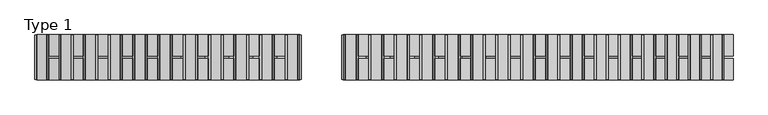
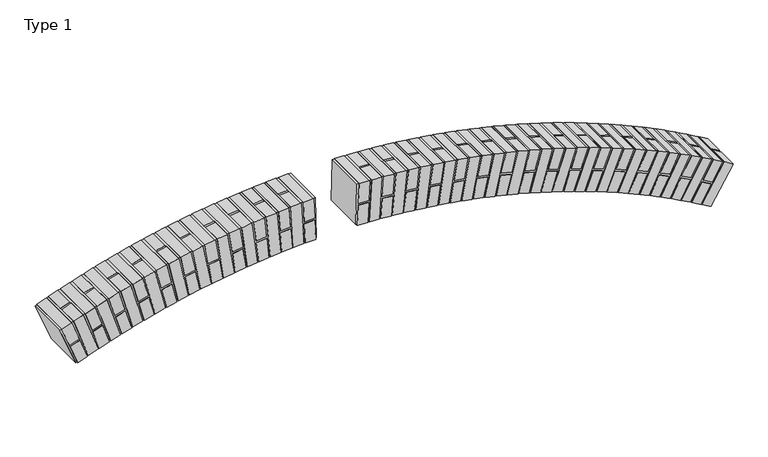
"""IFC4 building model written with IfcOpenShell, lengths in millimetres: proxy geometry, 00_GM_toog : Type 1."""

from ifc_helpers import new_model, si_unit, frame, origin, place, context, project, spatial, polyline, outline, extrude, source, transform, mapped, element, save


def type_1_8e1217ef(model_context):
    return source(origin(), model_context, "Body", "SweptSolid", [
        extrude(outline(polyline([(-33.5304655, 169.1537184), (-33.3801263, 159.6073904), (-133.2870305, 155.2934022), (-131.1300364, 105.3399501), (-31.2231322, 109.6539383), (-30.8114489, 100.1198354), (-235.8183922, 94.5699935), (-236.1881102, 100.8035341), (-141.1349511, 104.9079371), (-143.2919452, 154.8613892), (-237.8024787, 150.7804168), (-238.1723291, 157.0161892), (-33.5304655, 169.1537184)])), frame((0.0, 2.5, 0.0), z_axis=(0.0, 1.0, 0.0), x_axis=(0.0, 0.0, 1.0)), (0.0, 0.0, 1.0), 205.0),
        extrude(outline(polyline([(0.0, 50.0), (210.0, 50.0), (210.0, 0.0), (0.0, 0.0), (0.0, 50.0)])), frame((105.3399501, 210.0, -131.1300364), z_axis=(0.04313988139115512, 0.0, 0.9990690419753567), x_axis=(0.0, -1.0, 0.0)), (0.0, 0.0, 1.0), 100.0),
        extrude(outline(polyline([(0.0, 50.0), (210.0, 50.0), (210.0, 0.0), (0.0, 0.0), (0.0, 50.0)])), frame((100.593949, 210.0, -241.0418553), z_axis=(0.04313988139115512, 0.0, 0.9990690419753567), x_axis=(0.0, -1.0, 0.0)), (0.0, 0.0, 1.0), 100.0),
        extrude(outline(polyline([(210.0, 50.0), (210.0, 0.0), (110.0, 0.0), (110.0, 50.0), (210.0, 50.0)])), frame((206.6325287, 0.0, -246.1224192), z_axis=(0.05920702828123627, 0.0, 0.998245725160947), x_axis=(0.0, 1.0, 0.0)), (0.0, 0.0, 1.0), 210.0),
        extrude(outline(polyline([(100.0, 50.0), (100.0, 0.0), (0.0, 0.0), (0.0, 50.0), (100.0, 50.0)])), frame((206.6325287, 0.0, -246.1224192), z_axis=(0.05920702828123627, 0.0, 0.998245725160947), x_axis=(0.0, 1.0, 0.0)), (0.0, 0.0, 1.0), 210.0),
        extrude(outline(polyline([(-40.8857504, 287.9862039), (-40.4283717, 278.449654), (-140.1447749, 270.9237689), (-136.3818323, 221.0655673), (-36.6654292, 228.5914524), (-35.947235, 219.075529), (-240.6695155, 206.9332303), (-241.2395829, 213.1516499), (-146.3676698, 220.3119073), (-150.1306123, 270.1701089), (-244.4609345, 263.0507269), (-245.0312061, 269.271373), (-40.8857504, 287.9862039)])), frame((0.0, 2.5, 0.0), z_axis=(0.0, 1.0, 0.0), x_axis=(0.0, 0.0, 1.0)), (0.0, 0.0, 1.0), 205.0),
        extrude(outline(polyline([(0.0, 50.0), (210.0, 50.0), (210.0, 0.0), (0.0, 0.0), (0.0, 50.0)])), frame((221.0655673, 210.0, -136.3818323), z_axis=(0.0752588505534319, 0.0, 0.9971640313475895), x_axis=(0.0, -1.0, 0.0)), (0.0, 0.0, 1.0), 100.0),
        extrude(outline(polyline([(0.0, 50.0), (210.0, 50.0), (210.0, 0.0), (0.0, 0.0), (0.0, 50.0)])), frame((212.7860223, 210.0, -246.084073), z_axis=(0.0752588505534319, 0.0, 0.9971640313475895), x_axis=(0.0, -1.0, 0.0)), (0.0, 0.0, 1.0), 100.0),
        extrude(outline(polyline([(210.0, 50.0), (210.0, 0.0), (110.0, 0.0), (110.0, 50.0), (210.0, 50.0)])), frame((318.6062653, 0.0, -254.5734006), z_axis=(0.09129119349759061, 0.0, 0.9958242405112387), x_axis=(0.0, 1.0, 0.0)), (0.0, 0.0, 1.0), 210.0),
        extrude(outline(polyline([(100.0, 50.0), (100.0, 0.0), (0.0, 0.0), (0.0, 50.0), (100.0, 50.0)])), frame((318.6062653, 0.0, -254.5734006), z_axis=(0.09129119349759061, 0.0, 0.9958242405112387), x_axis=(0.0, 1.0, 0.0)), (0.0, 0.0, 1.0), 210.0),
        extrude(outline(polyline([(-52.0602176, 406.5205496), (-51.296273, 397.0036505), (-150.7189429, 386.2736598), (-145.3539475, 336.5623248), (-45.9312776, 347.2923156), (-44.907316, 337.8044231), (-249.1329934, 319.0822379), (-249.9028201, 325.279099), (-155.3103699, 335.4877981), (-160.6753652, 385.199133), (-254.7278199, 375.0487119), (-255.4979222, 381.2477916), (-52.0602176, 406.5205496)])), frame((0.0, 2.5, 0.0), z_axis=(0.0, 1.0, 0.0), x_axis=(0.0, 0.0, 1.0)), (0.0, 0.0, 1.0), 205.0),
        extrude(outline(polyline([(0.0, 50.0), (210.0, 50.0), (210.0, 0.0), (0.0, 0.0), (0.0, 50.0)])), frame((336.5623248, 210.0, -145.3539475), z_axis=(0.10729990744537966, 0.0, 0.9942266994313786), x_axis=(0.0, -1.0, 0.0)), (0.0, 0.0, 1.0), 100.0),
        extrude(outline(polyline([(0.0, 50.0), (210.0, 50.0), (210.0, 0.0), (0.0, 0.0), (0.0, 50.0)])), frame((324.7578073, 210.0, -254.7330398), z_axis=(0.10729990744537966, 0.0, 0.9942266994313786), x_axis=(0.0, -1.0, 0.0)), (0.0, 0.0, 1.0), 100.0),
        extrude(outline(polyline([(210.0, 50.0), (210.0, 0.0), (110.0, 0.0), (110.0, 50.0), (210.0, 50.0)])), frame((430.2501625, 0.0, -266.6223426), z_axis=(0.12328084884442252, 0.0, 0.9923718216012578), x_axis=(0.0, 1.0, 0.0)), (0.0, 0.0, 1.0), 210.0),
        extrude(outline(polyline([(100.0, 50.0), (100.0, 0.0), (0.0, 0.0), (0.0, 50.0), (100.0, 50.0)])), frame((430.2501625, 0.0, -266.6223426), z_axis=(0.12328084884442252, 0.0, 0.9923718216012578), x_axis=(0.0, 1.0, 0.0)), (0.0, 0.0, 1.0), 210.0),
        extrude(outline(polyline([(-67.0422986, 524.634042), (-65.9725789, 515.1466462), (-164.9985876, 501.2236581), (-158.0370935, 451.7106537), (-59.0110848, 465.6336418), (-57.6824158, 456.1836027), (-261.2000642, 430.9009134), (-262.1688531, 437.0698005), (-167.9537933, 450.3163726), (-174.9152873, 499.829377), (-268.592506, 486.658425), (-269.5616418, 492.8295207), (-67.0422986, 524.634042)])), frame((0.0, 2.5, 0.0), z_axis=(0.0, 1.0, 0.0), x_axis=(0.0, 0.0, 1.0)), (0.0, 0.0, 1.0), 205.0),
        extrude(outline(polyline([(0.0, 50.0), (210.0, 50.0), (210.0, 0.0), (0.0, 0.0), (0.0, 50.0)])), frame((451.7106537, 210.0, -158.0370935), z_axis=(0.1392298813307013, 0.0, 0.990260087120873), x_axis=(0.0, -1.0, 0.0)), (0.0, 0.0, 1.0), 100.0),
        extrude(outline(polyline([(0.0, 49.9999999), (210.0, 49.9999999), (210.0, 0.0), (0.0, 0.0), (0.0, 49.9999999)])), frame((436.3933845, 210.0, -266.979802), z_axis=(0.1392298813307013, 0.0, 0.990260087120873), x_axis=(0.0, -1.0, 0.0)), (0.0, 0.0, 1.0), 100.0),
        extrude(outline(polyline([(210.0, 50.0), (210.0, 0.0), (110.0, 0.0), (110.0, 50.0), (210.0, 50.0)])), frame((541.44864, 0.0, -282.2567714), z_axis=(0.15514287679925243, 0.0, 0.9878920425726953), x_axis=(0.0, 1.0, 0.0)), (0.0, 0.0, 1.0), 210.0),
        extrude(outline(polyline([(100.0, 50.0), (100.0, 0.0), (0.0, 0.0), (0.0, 50.0), (100.0, 50.0)])), frame((541.44864, 0.0, -282.2567714), z_axis=(0.15514287679925243, 0.0, 0.9878920425726953), x_axis=(0.0, 1.0, 0.0)), (0.0, 0.0, 1.0), 210.0),
        extrude(outline(polyline([(-85.8164831, 642.2044032), (-84.4420957, 632.7563326), (-182.9689258, 615.6547609), (-174.41814, 566.3913459), (-75.8913099, 583.4929175), (-74.2593091, 574.090515), (-276.8582352, 542.2734956), (-278.0249835, 548.4080224), (-184.2848508, 564.6787539), (-192.8356366, 613.9421689), (-286.0406393, 597.7643214), (-287.2078054, 603.9010445), (-85.8164831, 642.2044032)])), frame((0.0, 2.5, 0.0), z_axis=(0.0, 1.0, 0.0), x_axis=(0.0, 0.0, 1.0)), (0.0, 0.0, 1.0), 205.0),
        extrude(outline(polyline([(0.0, 50.0), (210.0, 50.0), (210.0, 0.0), (0.0, 0.0), (0.0, 50.0)])), frame((566.3913459, 210.0, -174.41814), z_axis=(0.17101571647257813, 0.0, 0.9852683008802073), x_axis=(0.0, -1.0, 0.0)), (0.0, 0.0, 1.0), 100.0),
        extrude(outline(polyline([(0.0, 50.0000001), (210.0, 50.0000001), (210.0, 0.0), (0.0, 0.0), (0.0, 50.0000001)])), frame((547.5771822, 210.0, -282.8116809), z_axis=(0.17101571647257813, 0.0, 0.9852683008802073), x_axis=(0.0, -1.0, 0.0)), (0.0, 0.0, 1.0), 100.0),
        extrude(outline(polyline([(210.0, 50.0), (210.0, 0.0), (110.0, 0.0), (110.0, 50.0), (210.0, 50.0)])), frame((652.086579, 0.0, -301.4605014), z_axis=(0.186844291966782, 0.0, 0.982389541149249), x_axis=(0.0, 1.0, 0.0)), (0.0, 0.0, 1.0), 210.0),
        extrude(outline(polyline([(100.0, 50.0), (100.0, 0.0), (0.0, 0.0), (0.0, 50.0), (100.0, 50.0)])), frame((652.086579, 0.0, -301.4605014), z_axis=(0.186844291966782, 0.0, 0.982389541149249), x_axis=(0.0, 1.0, 0.0)), (0.0, 0.0, 1.0), 210.0),
        extrude(outline(polyline([(-108.363335, 759.1099176), (-106.6857028, 749.7109533), (-204.6113536, 729.4485027), (-194.4801283, 680.4856773), (-96.5544775, 700.7481279), (-94.6208344, 691.4030958), (-296.0912962, 653.0846852), (-297.454796, 659.1785008), (-204.2866356, 678.4565473), (-214.4178609, 727.4193728), (-307.0541565, 708.251378), (-308.4181444, 714.3473753), (-108.363335, 759.1099176)])), frame((0.0, 2.5, 0.0), z_axis=(0.0, 1.0, 0.0), x_axis=(0.0, 0.0, 1.0)), (0.0, 0.0, 1.0), 205.0),
        extrude(outline(polyline([(0.0, 50.0), (210.0, 50.0), (210.0, 0.0), (0.0, 0.0), (0.0, 50.0)])), frame((680.4856773, 210.0, -194.4801283), z_axis=(0.20262450635487594, 0.0, 0.9792565084922555), x_axis=(0.0, -1.0, 0.0)), (0.0, 0.0, 1.0), 100.0),
        extrude(outline(polyline([(0.0, 50.0), (210.0, 50.0), (210.0, 0.0), (0.0, 0.0), (0.0, 50.0)])), frame((658.1940967, 210.0, -302.2122865), z_axis=(0.20262450635487594, 0.0, 0.9792565084922555), x_axis=(0.0, -1.0, 0.0)), (0.0, 0.0, 1.0), 100.0),
        extrude(outline(polyline([(210.0, 49.9999999), (210.0, 0.0), (110.0, 0.0), (110.0, 49.9999999), (210.0, 49.9999999)])), frame((762.0494405, 0.0, -324.2136517), z_axis=(0.21835227522726555, 0.0, 0.9758700138353861), x_axis=(0.0, 1.0, 0.0)), (0.0, 0.0, 1.0), 210.0),
        extrude(outline(polyline([(100.0, 49.9999999), (100.0, 0.0), (0.0, 0.0), (0.0, 49.9999999), (100.0, 49.9999999)])), frame((762.0494405, 0.0, -324.2136517), z_axis=(0.21835227522726555, 0.0, 0.9758700138353861), x_axis=(0.0, 1.0, 0.0)), (0.0, 0.0, 1.0), 210.0),
        extrude(outline(polyline([(-134.6595125, 875.229558), (-132.6803722, 865.8894304), (-229.9034656, 842.4870776), (-218.2022892, 793.875531), (-120.9791959, 817.2778837), (-118.7459124, 807.9998966), (-318.8793361, 763.2197642), (-320.4381758, 769.26656), (-227.9384408, 791.5319638), (-239.6396171, 840.1435105), (-331.6113032, 818.0052122), (-333.1707009, 824.0541729), (-134.6595125, 875.229558)])), frame((0.0, 2.5, 0.0), z_axis=(0.0, 1.0, 0.0), x_axis=(0.0, 0.0, 1.0)), (0.0, 0.0, 1.0), 205.0),
        extrude(outline(polyline([(0.0, 49.9999999), (210.0, 49.9999999), (210.0, 0.0), (0.0, 0.0), (0.0, 49.9999999)])), frame((793.875531, 210.0, -218.2022892), z_axis=(0.2340235277488462, 0.0, 0.9722309337086458), x_axis=(0.0, -1.0, 0.0)), (0.0, 0.0, 1.0), 100.0),
        extrude(outline(polyline([(0.0, 50.0), (210.0, 50.0), (210.0, 0.0), (0.0, 0.0), (0.0, 50.0)])), frame((768.129611, 210.0, -325.1615341), z_axis=(0.2340235277488462, 0.0, 0.9722309337086458), x_axis=(0.0, -1.0, 0.0)), (0.0, 0.0, 1.0), 100.0),
        extrude(outline(polyline([(210.0, 50.0), (210.0, 0.0), (110.0, 0.0), (110.0, 50.0), (210.0, 50.0)])), frame((871.2233849, 0.0, -350.492667), z_axis=(0.24963420771274006, 0.0, 0.9683402100189957), x_axis=(0.0, 1.0, 0.0)), (0.0, 0.0, 1.0), 210.0),
        extrude(outline(polyline([(100.0, 50.0), (100.0, 0.0), (0.0, 0.0), (0.0, 50.0), (100.0, 50.0)])), frame((871.2233849, 0.0, -350.492667), z_axis=(0.24963420771274006, 0.0, 0.9683402100189957), x_axis=(0.0, 1.0, 0.0)), (0.0, 0.0, 1.0), 210.0),
        extrude(outline(polyline([(-164.6777923, 990.4431107), (-162.3991929, 981.1714892), (-258.8190779, 954.6534617), (-245.5600642, 906.4435193), (-149.1401792, 932.9615467), (-146.6095673, 923.7602096), (-345.1987634, 872.5647144), (-346.9513291, 878.5582304), (-255.2157805, 903.787941), (-268.4747942, 951.9978835), (-359.6866564, 926.9122005), (-361.4398495, 932.9078623), (-164.6777923, 990.4431107)])), frame((0.0, 2.5, 0.0), z_axis=(0.0, 1.0, 0.0), x_axis=(0.0, 0.0, 1.0)), (0.0, 0.0, 1.0), 205.0),
        extrude(outline(polyline([(0.0, 49.9999999), (210.0, 49.9999999), (210.0, 0.0), (0.0, 0.0), (0.0, 49.9999999)])), frame((906.4435193, 210.0, -245.5600642), z_axis=(0.2651802745900883, 0.0, 0.9641988498065767), x_axis=(0.0, -1.0, 0.0)), (0.0, 0.0, 1.0), 100.0),
        extrude(outline(polyline([(0.0, 50.0), (210.0, 50.0), (210.0, 0.0), (0.0, 0.0), (0.0, 50.0)])), frame((877.2699135, 210.0, -351.6356655), z_axis=(0.2651802745900883, 0.0, 0.9641988498065767), x_axis=(0.0, -1.0, 0.0)), (0.0, 0.0, 1.0), 100.0),
        extrude(outline(polyline([(210.0, 50.0), (210.0, 0.0), (110.0, 0.0), (110.0, 50.0), (210.0, 50.0)])), frame((979.495389, 0.0, -380.2703418), z_axis=(0.2806577045759451, 0.0, 0.9598079249840363), x_axis=(0.0, 1.0, 0.0)), (0.0, 0.0, 1.0), 210.0),
        extrude(outline(polyline([(100.0, 50.0), (100.0, 0.0), (0.0, 0.0), (0.0, 50.0), (100.0, 50.0)])), frame((979.495389, 0.0, -380.2703418), z_axis=(0.2806577045759451, 0.0, 0.9598079249840363), x_axis=(0.0, 1.0, 0.0)), (0.0, 0.0, 1.0), 210.0),
        extrude(outline(polyline([(-198.3870978, 1104.6312999), (-195.8113982, 1095.4377831), (-291.3282554, 1065.8315339), (-276.5251308, 1018.0731053), (-181.0082736, 1047.6793545), (-178.1829531, 1038.5641932), (-375.0223307, 981.0063356), (-376.9668081, 986.940367), (-286.0904158, 1015.1082652), (-300.8935404, 1062.8666938), (-391.2511509, 1034.8595963), (-393.1963244, 1040.7957522), (-198.3870978, 1104.6312999)])), frame((0.0, 2.5, 0.0), z_axis=(0.0, 1.0, 0.0), x_axis=(0.0, 0.0, 1.0)), (0.0, 0.0, 1.0), 205.0),
        extrude(outline(polyline([(0.0, 50.0), (210.0, 50.0), (210.0, 0.0), (0.0, 0.0), (0.0, 50.0)])), frame((1018.0731053, 210.0, -276.5251308), z_axis=(0.2960624916306871, 0.0, 0.9551685720591049), x_axis=(0.0, -1.0, 0.0)), (0.0, 0.0, 1.0), 100.0),
        extrude(outline(polyline([(0.0, 50.0), (210.0, 50.0), (210.0, 0.0), (0.0, 0.0), (0.0, 50.0)])), frame((985.502016, 210.0, -381.607273), z_axis=(0.2960624916306871, 0.0, 0.9551685720591049), x_axis=(0.0, -1.0, 0.0)), (0.0, 0.0, 1.0), 100.0),
        extrude(outline(polyline([(210.0, 50.0), (210.0, 0.0), (110.0, 0.0), (110.0, 50.0), (210.0, 50.0)])), frame((1086.7533633, 0.0, -413.5158485), z_axis=(0.3113906485169718, 0.0, 0.9502819918404114), x_axis=(0.0, 1.0, 0.0)), (0.0, 0.0, 1.0), 210.0),
        extrude(outline(polyline([(100.0, 50.0), (100.0, 0.0), (0.0, 0.0), (0.0, 50.0), (100.0, 50.0)])), frame((1086.7533633, 0.0, -413.5158485), z_axis=(0.3113906485169718, 0.0, 0.9502819918404114), x_axis=(0.0, 1.0, 0.0)), (0.0, 0.0, 1.0), 210.0),
        extrude(outline(polyline([(-235.752531, 1217.6759116), (-232.8823978, 1208.5700171), (-327.3973427, 1175.9061963), (-311.0654323, 1128.6487238), (-216.5504874, 1161.3125446), (-213.4333832, 1152.2929957), (-408.319163, 1088.4323629), (-410.4535391, 1094.3007664), (-320.5303834, 1125.3776912), (-336.8622938, 1172.6351637), (-426.2721093, 1141.7356462), (-428.4072495, 1147.6061507), (-235.752531, 1217.6759116)])), frame((0.0, 2.5, 0.0), z_axis=(0.0, 1.0, 0.0), x_axis=(0.0, 0.0, 1.0)), (0.0, 0.0, 1.0), 205.0),
        extrude(outline(polyline([(0.0, 50.0), (210.0, 50.0), (210.0, 0.0), (0.0, 0.0), (0.0, 50.0)])), frame((1128.6487238, 210.0, -311.0654323), z_axis=(0.32663820783169173, 0.0, 0.945149449126698), x_axis=(0.0, -1.0, 0.0)), (0.0, 0.0, 1.0), 100.0),
        extrude(outline(polyline([(0.0, 50.0), (210.0, 50.0), (210.0, 0.0), (0.0, 0.0), (0.0, 50.0)])), frame((1092.7138704, 210.0, -415.0453283), z_axis=(0.32663820783169173, 0.0, 0.945149449126698), x_axis=(0.0, -1.0, 0.0)), (0.0, 0.0, 1.0), 100.0),
        extrude(outline(polyline([(210.0, 50.0), (210.0, 0.0), (110.0, 0.0), (110.0, 50.0), (210.0, 50.0)])), frame((1192.8862684, 0.0, -450.1947694), z_axis=(0.3418012230329286, 0.0, 0.9397722723794283), x_axis=(0.0, 1.0, 0.0)), (0.0, 0.0, 1.0), 210.0),
        extrude(outline(polyline([(100.0, 50.0), (100.0, 0.0), (0.0, 0.0), (0.0, 50.0), (100.0, 50.0)])), frame((1192.8862684, 0.0, -450.1947694), z_axis=(0.3418012230329286, 0.0, 0.9397722723794283), x_axis=(0.0, 1.0, 0.0)), (0.0, 0.0, 1.0), 210.0),
        extrude(outline(polyline([(-276.7354093, 1329.4599155), (-273.5738137, 1320.4510702), (-366.9889991, 1284.7634932), (-349.1452106, 1238.0559006), (-255.7300253, 1273.7434775), (-252.3243644, 1264.8288786), (-445.0547893, 1194.7315828), (-447.3768545, 1200.528283), (-358.5000292, 1234.4820618), (-376.3438176, 1281.1896545), (-464.7132759, 1247.429706), (-467.0361725, 1253.2284817), (-276.7354093, 1329.4599155)])), frame((0.0, 2.5, 0.0), z_axis=(0.0, 1.0, 0.0), x_axis=(0.0, 0.0, 1.0)), (0.0, 0.0, 1.0), 205.0),
        extrude(outline(polyline([(0.0, 49.9999999), (210.0, 49.9999999), (210.0, 0.0), (0.0, 0.0), (0.0, 49.9999999)])), frame((1238.0559006, 210.0, -349.1452106), z_axis=(0.3568757694613718, 0.0, 0.9341518533789642), x_axis=(0.0, -1.0, 0.0)), (0.0, 0.0, 1.0), 100.0),
        extrude(outline(polyline([(0.0, 50.0), (210.0, 50.0), (210.0, 0.0), (0.0, 0.0), (0.0, 50.0)])), frame((1198.7944849, 210.0, -451.9152145), z_axis=(0.3568757694613718, 0.0, 0.9341518533789642), x_axis=(0.0, -1.0, 0.0)), (0.0, 0.0, 1.0), 100.0),
        extrude(outline(polyline([(210.0, 50.0), (210.0, 0.0), (110.0, 0.0), (110.0, 50.0), (210.0, 50.0)])), frame((1297.7842293, 0.0, -490.2691324), z_axis=(0.3718579453562054, 0.0, 0.9282896468643079), x_axis=(0.0, 1.0, 0.0)), (0.0, 0.0, 1.0), 210.0),
        extrude(outline(polyline([(100.0, 50.0), (100.0, 0.0), (0.0, 0.0), (0.0, 50.0), (100.0, 50.0)])), frame((1297.7842293, 0.0, -490.2691324), z_axis=(0.3718579453562054, 0.0, 0.9282896468643079), x_axis=(0.0, 1.0, 0.0)), (0.0, 0.0, 1.0), 210.0),
        extrude(outline(polyline([(-321.2933048, 1439.8675863), (-317.8435199, 1430.9651168), (-410.0622369, 1392.2907295), (-390.7250433, 1346.181371), (-298.5063263, 1384.8557583), (-294.8156345, 1376.0553381), (-485.1911791, 1299.7939481), (-487.6985293, 1305.512944), (-399.9600447, 1342.308426), (-419.2972383, 1388.4177845), (-506.5348544, 1351.8323552), (-509.0431023, 1357.5533987), (-321.2933048, 1439.8675863)])), frame((0.0, 2.5, 0.0), z_axis=(0.0, 1.0, 0.0), x_axis=(0.0, 0.0, 1.0)), (0.0, 0.0, 1.0), 205.0),
        extrude(outline(polyline([(0.0, 50.0), (210.0, 50.0), (210.0, 0.0), (0.0, 0.0), (0.0, 50.0)])), frame((1346.181371, 210.0, -390.7250433), z_axis=(0.38674387286495593, 0.0, 0.9221871701565875), x_axis=(0.0, -1.0, 0.0)), (0.0, 0.0, 1.0), 100.0),
        extrude(outline(polyline([(0.0, 50.0), (210.0, 50.0), (210.0, 0.0), (0.0, 0.0), (0.0, 50.0)])), frame((1303.6340387, 210.0, -492.1787617), z_axis=(0.38674387286495593, 0.0, 0.9221871701565875), x_axis=(0.0, -1.0, 0.0)), (0.0, 0.0, 1.0), 100.0),
        extrude(outline(polyline([(210.0, 50.0), (210.0, 0.0), (110.0, 0.0), (110.0, 50.0), (210.0, 50.0)])), frame((1401.3386497, 0.0, -533.6974503), z_axis=(0.40152969904724134, 0.0, 0.9158460027663122), x_axis=(0.0, 1.0, 0.0)), (0.0, 0.0, 1.0), 210.0),
        extrude(outline(polyline([(100.0, 50.0), (100.0, 0.0), (0.0, 0.0), (0.0, 50.0), (100.0, 50.0)])), frame((1401.3386497, 0.0, -533.6974503), z_axis=(0.40152969904724134, 0.0, 0.9158460027663122), x_axis=(0.0, 1.0, 0.0)), (0.0, 0.0, 1.0), 210.0),
        extrude(outline(polyline([(-369.3800886, 1548.7846238), (-365.6456858, 1539.9977463), (-456.5724644, 1498.3765867), (-435.7618846, 1452.9131974), (-344.835106, 1494.534357), (-340.8632042, 1485.8572264), (-528.6867806, 1403.5106923), (-531.3768203, 1409.1460633), (-444.8675082, 1448.7451556), (-465.678088, 1494.2085449), (-551.6935484, 1454.8355101), (-554.3845512, 1460.4728988), (-369.3800886, 1548.7846238)])), frame((0.0, 2.5, 0.0), z_axis=(0.0, 1.0, 0.0), x_axis=(0.0, 0.0, 1.0)), (0.0, 0.0, 1.0), 205.0),
        extrude(outline(polyline([(0.0, 50.0), (210.0, 50.0), (210.0, 0.0), (0.0, 0.0), (0.0, 50.0)])), frame((1452.9131974, 210.0, -435.7618846), z_axis=(0.4162115968719885, 0.0, 0.9092677859845631), x_axis=(0.0, -1.0, 0.0)), (0.0, 0.0, 1.0), 100.0),
        extrude(outline(polyline([(0.0, 50.0), (210.0, 50.0), (210.0, 0.0), (0.0, 0.0), (0.0, 50.0)])), frame((1407.1239959, 210.0, -535.7942868), z_axis=(0.4162115968719885, 0.0, 0.9092677859845631), x_axis=(0.0, -1.0, 0.0)), (0.0, 0.0, 1.0), 100.0),
        extrude(outline(polyline([(210.0, 50.0000001), (210.0, 0.0), (110.0, 0.0), (110.0, 50.0000001), (210.0, 50.0000001)])), frame((1503.4423241, 0.0, -580.4347636), z_axis=(0.43078576620803966, 0.0, 0.9024542224581545), x_axis=(0.0, 1.0, 0.0)), (0.0, 0.0, 1.0), 210.0),
        extrude(outline(polyline([(100.0, 50.0000001), (100.0, 0.0), (0.0, 0.0), (0.0, 50.0000001), (100.0, 50.0000001)])), frame((1503.4423241, 0.0, -580.4347636), z_axis=(0.43078576620803966, 0.0, 0.9024542224581545), x_axis=(0.0, 1.0, 0.0)), (0.0, 0.0, 1.0), 210.0),
        extrude(outline(polyline([(-420.9459785, 1656.0982709), (-416.9308239, 1647.4360821), (-506.4715315, 1602.9112386), (-484.2091098, 1558.1408848), (-394.6684022, 1602.6657283), (-390.4194022, 1594.1208702), (-575.4965649, 1505.7744419), (-578.366509, 1511.3203539), (-493.1759289, 1553.6820612), (-515.4383507, 1598.452415), (-600.1426072, 1556.3325361), (-603.0135789, 1561.8804337), (-420.9459785, 1656.0982709)])), frame((0.0, 2.5, 0.0), z_axis=(0.0, 1.0, 0.0), x_axis=(0.0, 0.0, 1.0)), (0.0, 0.0, 1.0), 205.0),
        extrude(outline(polyline([(0.0, 50.0), (210.0, 50.0), (210.0, 0.0), (0.0, 0.0), (0.0, 50.0)])), frame((1558.1408848, 210.0, -484.2091098), z_axis=(0.4452484348076845, 0.0, 0.8954070757489618), x_axis=(0.0, -1.0, 0.0)), (0.0, 0.0, 1.0), 100.0),
        extrude(outline(polyline([(0.0, 49.9999999), (210.0, 49.9999999), (210.0, 0.0), (0.0, 0.0), (0.0, 49.9999999)])), frame((1509.1572178, 210.0, -582.7166365), z_axis=(0.4452484348076845, 0.0, 0.8954070757489618), x_axis=(0.0, -1.0, 0.0)), (0.0, 0.0, 1.0), 100.0),
        extrude(outline(polyline([(210.0, 50.0), (210.0, 0.0), (110.0, 0.0), (110.0, 50.0), (210.0, 50.0)])), frame((1603.9895489, 0.0, -630.4326871), z_axis=(0.4595958592830959, 0.0, 0.8881281698774298), x_axis=(0.0, 1.0, 0.0)), (0.0, 0.0, 1.0), 210.0),
        extrude(outline(polyline([(100.0, 50.0), (100.0, 0.0), (0.0, 0.0), (0.0, 50.0), (100.0, 50.0)])), frame((1603.9895489, 0.0, -630.4326871), z_axis=(0.4595958592830959, 0.0, 0.8881281698774298), x_axis=(0.0, 1.0, 0.0)), (0.0, 0.0, 1.0), 210.0),
        extrude(outline(polyline([(-475.9375905, 1761.6974301), (-471.6458409, 1753.1688977), (-559.7077798, 1705.7864651), (-536.0165635, 1661.7554957), (-447.9546246, 1709.1379283), (-443.4329252, 1700.7341889), (-625.5720717, 1606.4793275), (-628.6189492, 1611.9300392), (-544.8352952, 1657.0105063), (-568.5265115, 1701.0414757), (-651.8318736, 1656.2183574), (-654.879842, 1661.6710206), (-475.9375905, 1761.6974301)])), frame((0.0, 2.5, 0.0), z_axis=(0.0, 1.0, 0.0), x_axis=(0.0, 0.0, 1.0)), (0.0, 0.0, 1.0), 205.0),
        extrude(outline(polyline([(0.0, 50.0), (210.0, 50.0), (210.0, 0.0), (0.0, 0.0), (0.0, 50.0)])), frame((1661.7554957, 210.0, -536.0165635), z_axis=(0.47382432607517866, 0.0, 0.8806193888504856), x_axis=(0.0, -1.0, 0.0)), (0.0, 0.0, 1.0), 100.0),
        extrude(outline(polyline([(0.0, 50.0), (210.0, 50.0), (210.0, 0.0), (0.0, 0.0), (0.0, 50.0)])), frame((1609.6280737, 210.0, -632.8972341), z_axis=(0.47382432607517866, 0.0, 0.8806193888504856), x_axis=(0.0, -1.0, 0.0)), (0.0, 0.0, 1.0), 100.0),
        extrude(outline(polyline([(210.0, 50.0), (210.0, 0.0), (110.0, 0.0), (110.0, 50.0), (210.0, 50.0)])), frame((1702.8762319, 0.0, -683.6394602), z_axis=(0.4879301524148094, 0.0, 0.8728826761738722), x_axis=(0.0, 1.0, 0.0)), (0.0, 0.0, 1.0), 210.0),
        extrude(outline(polyline([(100.0, 50.0), (100.0, 0.0), (0.0, 0.0), (0.0, 50.0), (100.0, 50.0)])), frame((1702.8762319, 0.0, -683.6394602), z_axis=(0.4879301524148094, 0.0, 0.8728826761738722), x_axis=(0.0, 1.0, 0.0)), (0.0, 0.0, 1.0), 210.0),
        extrude(outline(polyline([(-534.2979943, 1865.4727794), (-529.7340926, 1857.0867325), (-616.2260961, 1806.8957638), (-591.1306117, 1763.6497621), (-504.6386083, 1813.8407308), (-499.8488907, 1805.5868102), (-678.86146, 1705.5210939), (-682.0821166, 1710.8709622), (-599.7921264, 1758.6235192), (-624.8876108, 1801.8695209), (-706.7078359, 1754.3895668), (-709.9296455, 1759.7413505), (-534.2979943, 1865.4727794)])), frame((0.0, 2.5, 0.0), z_axis=(0.0, 1.0, 0.0), x_axis=(0.0, 0.0, 1.0)), (0.0, 0.0, 1.0), 205.0),
        extrude(outline(polyline([(0.0, 50.0), (210.0, 50.0), (210.0, 0.0), (0.0, 0.0), (0.0, 50.0)])), frame((1763.6497621, 210.0, -591.1306117), z_axis=(0.5019096872759921, 0.0, 0.864920034349139), x_axis=(0.0, -1.0, 0.0)), (0.0, 0.0, 1.0), 100.0),
        extrude(outline(polyline([(0.0, 50.0), (210.0, 50.0), (210.0, 0.0), (0.0, 0.0), (0.0, 50.0)])), frame((1708.4325505, 210.0, -686.2841298), z_axis=(0.5019096872759921, 0.0, 0.864920034349139), x_axis=(0.0, -1.0, 0.0)), (0.0, 0.0, 1.0), 100.0),
        extrude(outline(polyline([(210.0, 50.0), (210.0, 0.0), (110.0, 0.0), (110.0, 50.0), (210.0, 50.0)])), frame((1800.0, 0.0, -740.0), z_axis=(0.5157593123209204, 0.0, 0.8567335243552988), x_axis=(0.0, 1.0, 0.0)), (0.0, 0.0, 1.0), 210.0),
        extrude(outline(polyline([(100.0, 50.0), (100.0, 0.0), (0.0, 0.0), (0.0, 50.0), (100.0, 50.0)])), frame((1800.0, 0.0, -740.0), z_axis=(0.5157593123209204, 0.0, 0.8567335243552988), x_axis=(0.0, 1.0, 0.0)), (0.0, 0.0, 1.0), 210.0),
        extrude(outline(polyline([(-33.5304655, -169.1537184), (-238.1723291, -157.0161892), (-237.8024787, -150.7804168), (-143.2919452, -154.8613892), (-141.1349511, -104.9079371), (-236.1881102, -100.8035341), (-235.8183922, -94.5699935), (-30.8114489, -100.1198354), (-31.2231322, -109.6539383), (-131.1300364, -105.3399501), (-133.2870305, -155.2934022), (-33.3801263, -159.6073904), (-33.5304655, -169.1537184)])), frame((0.0, 2.5, 0.0), z_axis=(0.0, 1.0, 0.0), x_axis=(0.0, 0.0, 1.0)), (0.0, 0.0, 1.0), 205.0),
        extrude(outline(polyline([(0.0, -50.0), (0.0, 0.0), (210.0, 0.0), (210.0, -50.0), (0.0, -50.0)])), frame((-105.3399501, 210.0, -131.1300364), z_axis=(-0.04313988139115512, 0.0, 0.9990690419753567), x_axis=(0.0, -1.0, 0.0)), (0.0, 0.0, 1.0), 100.0),
        extrude(outline(polyline([(0.0, -50.0), (0.0, 0.0), (210.0, 0.0), (210.0, -50.0), (0.0, -50.0)])), frame((-100.593949, 210.0, -241.0418553), z_axis=(-0.04313988139115512, 0.0, 0.9990690419753567), x_axis=(0.0, -1.0, 0.0)), (0.0, 0.0, 1.0), 100.0),
        extrude(outline(polyline([(210.0, -50.0), (110.0, -50.0), (110.0, 0.0), (210.0, 0.0), (210.0, -50.0)])), frame((-206.6325287, 0.0, -246.1224192), z_axis=(-0.05920702828123627, 0.0, 0.998245725160947), x_axis=(0.0, 1.0, 0.0)), (0.0, 0.0, 1.0), 210.0),
        extrude(outline(polyline([(100.0, -50.0), (0.0, -50.0), (0.0, 0.0), (100.0, 0.0), (100.0, -50.0)])), frame((-206.6325287, 0.0, -246.1224192), z_axis=(-0.05920702828123627, 0.0, 0.998245725160947), x_axis=(0.0, 1.0, 0.0)), (0.0, 0.0, 1.0), 210.0),
        extrude(outline(polyline([(-40.8857504, -287.9862039), (-245.0312061, -269.271373), (-244.4609345, -263.0507269), (-150.1306123, -270.1701089), (-146.3676698, -220.3119073), (-241.2395829, -213.1516499), (-240.6695155, -206.9332303), (-35.947235, -219.075529), (-36.6654292, -228.5914524), (-136.3818323, -221.0655673), (-140.1447749, -270.9237689), (-40.4283717, -278.449654), (-40.8857504, -287.9862039)])), frame((0.0, 2.5, 0.0), z_axis=(0.0, 1.0, 0.0), x_axis=(0.0, 0.0, 1.0)), (0.0, 0.0, 1.0), 205.0),
        extrude(outline(polyline([(0.0, -50.0), (0.0, 0.0), (210.0, 0.0), (210.0, -50.0), (0.0, -50.0)])), frame((-221.0655673, 210.0, -136.3818323), z_axis=(-0.0752588505534319, 0.0, 0.9971640313475895), x_axis=(0.0, -1.0, 0.0)), (0.0, 0.0, 1.0), 100.0),
        extrude(outline(polyline([(0.0, -50.0), (0.0, 0.0), (210.0, 0.0), (210.0, -50.0), (0.0, -50.0)])), frame((-212.7860223, 210.0, -246.084073), z_axis=(-0.0752588505534319, 0.0, 0.9971640313475895), x_axis=(0.0, -1.0, 0.0)), (0.0, 0.0, 1.0), 100.0),
        extrude(outline(polyline([(210.0, -50.0), (110.0, -50.0), (110.0, 0.0), (210.0, 0.0), (210.0, -50.0)])), frame((-318.6062653, 0.0, -254.5734006), z_axis=(-0.09129119349759061, 0.0, 0.9958242405112387), x_axis=(0.0, 1.0, 0.0)), (0.0, 0.0, 1.0), 210.0),
        extrude(outline(polyline([(100.0, -50.0), (0.0, -50.0), (0.0, 0.0), (100.0, 0.0), (100.0, -50.0)])), frame((-318.6062653, 0.0, -254.5734006), z_axis=(-0.09129119349759061, 0.0, 0.9958242405112387), x_axis=(0.0, 1.0, 0.0)), (0.0, 0.0, 1.0), 210.0),
        extrude(outline(polyline([(-52.0602176, -406.5205496), (-255.4979222, -381.2477916), (-254.7278199, -375.0487119), (-160.6753652, -385.199133), (-155.3103699, -335.4877981), (-249.9028201, -325.279099), (-249.1329934, -319.0822379), (-44.907316, -337.8044231), (-45.9312776, -347.2923156), (-145.3539475, -336.5623248), (-150.7189429, -386.2736598), (-51.296273, -397.0036505), (-52.0602176, -406.5205496)])), frame((0.0, 2.5, 0.0), z_axis=(0.0, 1.0, 0.0), x_axis=(0.0, 0.0, 1.0)), (0.0, 0.0, 1.0), 205.0),
        extrude(outline(polyline([(0.0, -50.0), (0.0, 0.0), (210.0, 0.0), (210.0, -50.0), (0.0, -50.0)])), frame((-336.5623248, 210.0, -145.3539475), z_axis=(-0.10729990744537966, 0.0, 0.9942266994313786), x_axis=(0.0, -1.0, 0.0)), (0.0, 0.0, 1.0), 100.0),
        extrude(outline(polyline([(0.0, -50.0), (0.0, 0.0), (210.0, 0.0), (210.0, -50.0), (0.0, -50.0)])), frame((-324.7578073, 210.0, -254.7330398), z_axis=(-0.10729990744537966, 0.0, 0.9942266994313786), x_axis=(0.0, -1.0, 0.0)), (0.0, 0.0, 1.0), 100.0),
        extrude(outline(polyline([(210.0, -50.0), (110.0, -50.0), (110.0, 0.0), (210.0, 0.0), (210.0, -50.0)])), frame((-430.2501625, 0.0, -266.6223426), z_axis=(-0.12328084884442252, 0.0, 0.9923718216012578), x_axis=(0.0, 1.0, 0.0)), (0.0, 0.0, 1.0), 210.0),
        extrude(outline(polyline([(100.0, -50.0), (0.0, -50.0), (0.0, 0.0), (100.0, 0.0), (100.0, -50.0)])), frame((-430.2501625, 0.0, -266.6223426), z_axis=(-0.12328084884442252, 0.0, 0.9923718216012578), x_axis=(0.0, 1.0, 0.0)), (0.0, 0.0, 1.0), 210.0),
        extrude(outline(polyline([(-67.0422986, -524.634042), (-269.5616418, -492.8295207), (-268.592506, -486.658425), (-174.9152873, -499.829377), (-167.9537933, -450.3163726), (-262.1688531, -437.0698005), (-261.2000642, -430.9009134), (-57.6824158, -456.1836027), (-59.0110848, -465.6336418), (-158.0370935, -451.7106537), (-164.9985876, -501.2236581), (-65.9725789, -515.1466462), (-67.0422986, -524.634042)])), frame((0.0, 2.5, 0.0), z_axis=(0.0, 1.0, 0.0), x_axis=(0.0, 0.0, 1.0)), (0.0, 0.0, 1.0), 205.0),
        extrude(outline(polyline([(0.0, -50.0), (0.0, 0.0), (210.0, 0.0), (210.0, -50.0), (0.0, -50.0)])), frame((-451.7106537, 210.0, -158.0370935), z_axis=(-0.1392298813307013, 0.0, 0.990260087120873), x_axis=(0.0, -1.0, 0.0)), (0.0, 0.0, 1.0), 100.0),
        extrude(outline(polyline([(0.0, -49.9999999), (0.0, 0.0), (210.0, 0.0), (210.0, -49.9999999), (0.0, -49.9999999)])), frame((-436.3933845, 210.0, -266.979802), z_axis=(-0.1392298813307013, 0.0, 0.990260087120873), x_axis=(0.0, -1.0, 0.0)), (0.0, 0.0, 1.0), 100.0),
        extrude(outline(polyline([(210.0, -50.0), (110.0, -50.0), (110.0, 0.0), (210.0, 0.0), (210.0, -50.0)])), frame((-541.44864, 0.0, -282.2567714), z_axis=(-0.15514287679925243, 0.0, 0.9878920425726953), x_axis=(0.0, 1.0, 0.0)), (0.0, 0.0, 1.0), 210.0),
        extrude(outline(polyline([(100.0, -50.0), (0.0, -50.0), (0.0, 0.0), (100.0, 0.0), (100.0, -50.0)])), frame((-541.44864, 0.0, -282.2567714), z_axis=(-0.15514287679925243, 0.0, 0.9878920425726953), x_axis=(0.0, 1.0, 0.0)), (0.0, 0.0, 1.0), 210.0),
        extrude(outline(polyline([(-85.8164831, -642.2044032), (-287.2078054, -603.9010445), (-286.0406393, -597.7643214), (-192.8356366, -613.9421689), (-184.2848508, -564.6787539), (-278.0249835, -548.4080224), (-276.8582352, -542.2734956), (-74.2593091, -574.090515), (-75.8913099, -583.4929175), (-174.41814, -566.3913459), (-182.9689258, -615.6547609), (-84.4420957, -632.7563326), (-85.8164831, -642.2044032)])), frame((0.0, 2.5, 0.0), z_axis=(0.0, 1.0, 0.0), x_axis=(0.0, 0.0, 1.0)), (0.0, 0.0, 1.0), 205.0),
        extrude(outline(polyline([(0.0, -50.0), (0.0, 0.0), (210.0, 0.0), (210.0, -50.0), (0.0, -50.0)])), frame((-566.3913459, 210.0, -174.41814), z_axis=(-0.17101571647257813, 0.0, 0.9852683008802073), x_axis=(0.0, -1.0, 0.0)), (0.0, 0.0, 1.0), 100.0),
        extrude(outline(polyline([(0.0, -50.0000001), (0.0, 0.0), (210.0, 0.0), (210.0, -50.0000001), (0.0, -50.0000001)])), frame((-547.5771822, 210.0, -282.8116809), z_axis=(-0.17101571647257813, 0.0, 0.9852683008802073), x_axis=(0.0, -1.0, 0.0)), (0.0, 0.0, 1.0), 100.0),
        extrude(outline(polyline([(210.0, -50.0), (110.0, -50.0), (110.0, 0.0), (210.0, 0.0), (210.0, -50.0)])), frame((-652.086579, 0.0, -301.4605014), z_axis=(-0.186844291966782, 0.0, 0.982389541149249), x_axis=(0.0, 1.0, 0.0)), (0.0, 0.0, 1.0), 210.0),
        extrude(outline(polyline([(100.0, -50.0), (0.0, -50.0), (0.0, 0.0), (100.0, 0.0), (100.0, -50.0)])), frame((-652.086579, 0.0, -301.4605014), z_axis=(-0.186844291966782, 0.0, 0.982389541149249), x_axis=(0.0, 1.0, 0.0)), (0.0, 0.0, 1.0), 210.0),
        extrude(outline(polyline([(-108.363335, -759.1099176), (-308.4181444, -714.3473753), (-307.0541565, -708.251378), (-214.4178609, -727.4193728), (-204.2866356, -678.4565473), (-297.454796, -659.1785008), (-296.0912962, -653.0846852), (-94.6208344, -691.4030958), (-96.5544775, -700.7481279), (-194.4801283, -680.4856773), (-204.6113536, -729.4485027), (-106.6857028, -749.7109533), (-108.363335, -759.1099176)])), frame((0.0, 2.5, 0.0), z_axis=(0.0, 1.0, 0.0), x_axis=(0.0, 0.0, 1.0)), (0.0, 0.0, 1.0), 205.0),
        extrude(outline(polyline([(0.0, -50.0), (0.0, 0.0), (210.0, 0.0), (210.0, -50.0), (0.0, -50.0)])), frame((-680.4856773, 210.0, -194.4801283), z_axis=(-0.20262450635487594, 0.0, 0.9792565084922555), x_axis=(0.0, -1.0, 0.0)), (0.0, 0.0, 1.0), 100.0),
        extrude(outline(polyline([(0.0, -50.0), (0.0, 0.0), (210.0, 0.0), (210.0, -50.0), (0.0, -50.0)])), frame((-658.1940967, 210.0, -302.2122865), z_axis=(-0.20262450635487594, 0.0, 0.9792565084922555), x_axis=(0.0, -1.0, 0.0)), (0.0, 0.0, 1.0), 100.0),
        extrude(outline(polyline([(210.0, -49.9999999), (110.0, -49.9999999), (110.0, 0.0), (210.0, 0.0), (210.0, -49.9999999)])), frame((-762.0494405, 0.0, -324.2136517), z_axis=(-0.21835227522726555, 0.0, 0.9758700138353861), x_axis=(0.0, 1.0, 0.0)), (0.0, 0.0, 1.0), 210.0),
        extrude(outline(polyline([(100.0, -49.9999999), (0.0, -49.9999999), (0.0, 0.0), (100.0, 0.0), (100.0, -49.9999999)])), frame((-762.0494405, 0.0, -324.2136517), z_axis=(-0.21835227522726555, 0.0, 0.9758700138353861), x_axis=(0.0, 1.0, 0.0)), (0.0, 0.0, 1.0), 210.0),
        extrude(outline(polyline([(-134.6595125, -875.229558), (-333.1707009, -824.0541729), (-331.6113032, -818.0052122), (-239.6396171, -840.1435105), (-227.9384408, -791.5319638), (-320.4381758, -769.26656), (-318.8793361, -763.2197642), (-118.7459124, -807.9998966), (-120.9791959, -817.2778837), (-218.2022892, -793.875531), (-229.9034656, -842.4870776), (-132.6803722, -865.8894304), (-134.6595125, -875.229558)])), frame((0.0, 2.5, 0.0), z_axis=(0.0, 1.0, 0.0), x_axis=(0.0, 0.0, 1.0)), (0.0, 0.0, 1.0), 205.0),
        extrude(outline(polyline([(0.0, -49.9999999), (0.0, 0.0), (210.0, 0.0), (210.0, -49.9999999), (0.0, -49.9999999)])), frame((-793.875531, 210.0, -218.2022892), z_axis=(-0.2340235277488462, 0.0, 0.9722309337086458), x_axis=(0.0, -1.0, 0.0)), (0.0, 0.0, 1.0), 100.0),
        extrude(outline(polyline([(0.0, -50.0), (0.0, 0.0), (210.0, 0.0), (210.0, -50.0), (0.0, -50.0)])), frame((-768.129611, 210.0, -325.1615341), z_axis=(-0.2340235277488462, 0.0, 0.9722309337086458), x_axis=(0.0, -1.0, 0.0)), (0.0, 0.0, 1.0), 100.0),
        extrude(outline(polyline([(210.0, -50.0), (110.0, -50.0), (110.0, 0.0), (210.0, 0.0), (210.0, -50.0)])), frame((-871.2233849, 0.0, -350.492667), z_axis=(-0.24963420771274006, 0.0, 0.9683402100189957), x_axis=(0.0, 1.0, 0.0)), (0.0, 0.0, 1.0), 210.0),
        extrude(outline(polyline([(100.0, -50.0), (0.0, -50.0), (0.0, 0.0), (100.0, 0.0), (100.0, -50.0)])), frame((-871.2233849, 0.0, -350.492667), z_axis=(-0.24963420771274006, 0.0, 0.9683402100189957), x_axis=(0.0, 1.0, 0.0)), (0.0, 0.0, 1.0), 210.0),
        extrude(outline(polyline([(-164.6777923, -990.4431107), (-361.4398495, -932.9078623), (-359.6866564, -926.9122005), (-268.4747942, -951.9978835), (-255.2157805, -903.787941), (-346.9513291, -878.5582304), (-345.1987634, -872.5647144), (-146.6095673, -923.7602096), (-149.1401792, -932.9615467), (-245.5600642, -906.4435193), (-258.8190779, -954.6534617), (-162.3991929, -981.1714892), (-164.6777923, -990.4431107)])), frame((0.0, 2.5, 0.0), z_axis=(0.0, 1.0, 0.0), x_axis=(0.0, 0.0, 1.0)), (0.0, 0.0, 1.0), 205.0),
        extrude(outline(polyline([(0.0, -49.9999999), (0.0, 0.0), (210.0, 0.0), (210.0, -49.9999999), (0.0, -49.9999999)])), frame((-906.4435193, 210.0, -245.5600642), z_axis=(-0.2651802745900883, 0.0, 0.9641988498065767), x_axis=(0.0, -1.0, 0.0)), (0.0, 0.0, 1.0), 100.0),
        extrude(outline(polyline([(0.0, -50.0), (0.0, 0.0), (210.0, 0.0), (210.0, -50.0), (0.0, -50.0)])), frame((-877.2699135, 210.0, -351.6356655), z_axis=(-0.2651802745900883, 0.0, 0.9641988498065767), x_axis=(0.0, -1.0, 0.0)), (0.0, 0.0, 1.0), 100.0),
        extrude(outline(polyline([(210.0, -50.0), (110.0, -50.0), (110.0, 0.0), (210.0, 0.0), (210.0, -50.0)])), frame((-979.495389, 0.0, -380.2703418), z_axis=(-0.2806577045759451, 0.0, 0.9598079249840363), x_axis=(0.0, 1.0, 0.0)), (0.0, 0.0, 1.0), 210.0),
        extrude(outline(polyline([(100.0, -50.0), (0.0, -50.0), (0.0, 0.0), (100.0, 0.0), (100.0, -50.0)])), frame((-979.495389, 0.0, -380.2703418), z_axis=(-0.2806577045759451, 0.0, 0.9598079249840363), x_axis=(0.0, 1.0, 0.0)), (0.0, 0.0, 1.0), 210.0),
        extrude(outline(polyline([(-198.3870978, -1104.6312999), (-393.1963244, -1040.7957522), (-391.2511509, -1034.8595963), (-300.8935404, -1062.8666938), (-286.0904158, -1015.1082652), (-376.9668081, -986.940367), (-375.0223307, -981.0063356), (-178.1829531, -1038.5641932), (-181.0082736, -1047.6793545), (-276.5251308, -1018.0731053), (-291.3282554, -1065.8315339), (-195.8113982, -1095.4377831), (-198.3870978, -1104.6312999)])), frame((0.0, 2.5, 0.0), z_axis=(0.0, 1.0, 0.0), x_axis=(0.0, 0.0, 1.0)), (0.0, 0.0, 1.0), 205.0),
        extrude(outline(polyline([(0.0, -50.0), (0.0, 0.0), (210.0, 0.0), (210.0, -50.0), (0.0, -50.0)])), frame((-1018.0731053, 210.0, -276.5251308), z_axis=(-0.2960624916306871, 0.0, 0.9551685720591049), x_axis=(0.0, -1.0, 0.0)), (0.0, 0.0, 1.0), 100.0),
        extrude(outline(polyline([(0.0, -50.0), (0.0, 0.0), (210.0, 0.0), (210.0, -50.0), (0.0, -50.0)])), frame((-985.502016, 210.0, -381.607273), z_axis=(-0.2960624916306871, 0.0, 0.9551685720591049), x_axis=(0.0, -1.0, 0.0)), (0.0, 0.0, 1.0), 100.0),
        extrude(outline(polyline([(210.0, -50.0), (110.0, -50.0), (110.0, 0.0), (210.0, 0.0), (210.0, -50.0)])), frame((-1086.7533633, 0.0, -413.5158485), z_axis=(-0.3113906485169718, 0.0, 0.9502819918404114), x_axis=(0.0, 1.0, 0.0)), (0.0, 0.0, 1.0), 210.0),
        extrude(outline(polyline([(100.0, -50.0), (0.0, -50.0), (0.0, 0.0), (100.0, 0.0), (100.0, -50.0)])), frame((-1086.7533633, 0.0, -413.5158485), z_axis=(-0.3113906485169718, 0.0, 0.9502819918404114), x_axis=(0.0, 1.0, 0.0)), (0.0, 0.0, 1.0), 210.0),
        extrude(outline(polyline([(-235.752531, -1217.6759116), (-428.4072495, -1147.6061507), (-426.2721093, -1141.7356462), (-336.8622938, -1172.6351637), (-320.5303834, -1125.3776912), (-410.4535391, -1094.3007664), (-408.319163, -1088.4323629), (-213.4333832, -1152.2929957), (-216.5504874, -1161.3125446), (-311.0654323, -1128.6487238), (-327.3973427, -1175.9061963), (-232.8823978, -1208.5700171), (-235.752531, -1217.6759116)])), frame((0.0, 2.5, 0.0), z_axis=(0.0, 1.0, 0.0), x_axis=(0.0, 0.0, 1.0)), (0.0, 0.0, 1.0), 205.0),
        extrude(outline(polyline([(0.0, -50.0), (0.0, 0.0), (210.0, 0.0), (210.0, -50.0), (0.0, -50.0)])), frame((-1128.6487238, 210.0, -311.0654323), z_axis=(-0.32663820783169173, 0.0, 0.945149449126698), x_axis=(0.0, -1.0, 0.0)), (0.0, 0.0, 1.0), 100.0),
        extrude(outline(polyline([(0.0, -50.0), (0.0, 0.0), (210.0, 0.0), (210.0, -50.0), (0.0, -50.0)])), frame((-1092.7138704, 210.0, -415.0453283), z_axis=(-0.32663820783169173, 0.0, 0.945149449126698), x_axis=(0.0, -1.0, 0.0)), (0.0, 0.0, 1.0), 100.0),
        extrude(outline(polyline([(210.0, -50.0), (110.0, -50.0), (110.0, 0.0), (210.0, 0.0), (210.0, -50.0)])), frame((-1192.8862684, 0.0, -450.1947694), z_axis=(-0.3418012230329286, 0.0, 0.9397722723794283), x_axis=(0.0, 1.0, 0.0)), (0.0, 0.0, 1.0), 210.0),
        extrude(outline(polyline([(100.0, -50.0), (0.0, -50.0), (0.0, 0.0), (100.0, 0.0), (100.0, -50.0)])), frame((-1192.8862684, 0.0, -450.1947694), z_axis=(-0.3418012230329286, 0.0, 0.9397722723794283), x_axis=(0.0, 1.0, 0.0)), (0.0, 0.0, 1.0), 210.0),
        extrude(outline(polyline([(-276.7354093, -1329.4599155), (-467.0361725, -1253.2284817), (-464.7132759, -1247.429706), (-376.3438176, -1281.1896545), (-358.5000292, -1234.4820618), (-447.3768545, -1200.528283), (-445.0547893, -1194.7315828), (-252.3243644, -1264.8288786), (-255.7300253, -1273.7434775), (-349.1452106, -1238.0559006), (-366.9889991, -1284.7634932), (-273.5738137, -1320.4510702), (-276.7354093, -1329.4599155)])), frame((0.0, 2.5, 0.0), z_axis=(0.0, 1.0, 0.0), x_axis=(0.0, 0.0, 1.0)), (0.0, 0.0, 1.0), 205.0),
        extrude(outline(polyline([(0.0, -49.9999999), (0.0, 0.0), (210.0, 0.0), (210.0, -49.9999999), (0.0, -49.9999999)])), frame((-1238.0559006, 210.0, -349.1452106), z_axis=(-0.3568757694613718, 0.0, 0.9341518533789642), x_axis=(0.0, -1.0, 0.0)), (0.0, 0.0, 1.0), 100.0),
        extrude(outline(polyline([(0.0, -50.0), (0.0, 0.0), (210.0, 0.0), (210.0, -50.0), (0.0, -50.0)])), frame((-1198.7944849, 210.0, -451.9152145), z_axis=(-0.3568757694613718, 0.0, 0.9341518533789642), x_axis=(0.0, -1.0, 0.0)), (0.0, 0.0, 1.0), 100.0),
    ])


if __name__ == "__main__":
    model = new_model("IFC4")
    model_context = context("Model", 3, world=origin())
    ifc_project = project(units=[si_unit("LENGTHUNIT", "METRE", prefix="MILLI")], contexts=[model_context])
    site = spatial("IfcSite", under=ifc_project)
    building = spatial("IfcBuilding", under=site)
    placement = place(None, origin())
    type_1_shape = type_1_8e1217ef(model_context)
    element("IfcBuildingElementProxy", 1, Name="00_GM_toog : Type 1", ObjectType="00_GM_toog : Type 1", at=placement, inside=building, context=model_context, shape_type="MappedRepresentation", body=[
        mapped(type_1_shape, transform((0.0, 0.0, 0.0), x_axis=(1.0, 0.0, 0.0), y_axis=(0.0, 1.0, 0.0), z_axis=(0.0, 0.0, 1.0))),
    ])
    save(model, "model.ifc")

# Revit data of these elements
# Type "00_GM_toog : Type 1"
#   straal_hart_rollaag [instance default] = 1935 mm
#   straal_buitenlijn [instance default] = 2040 mm
#   straal [instance default] = 1830 mm
#   stootvoegbreedte_onderzijde [instance default] = 5 mm
#   offset [instance default] = -2070 mm
#   kop_voeg [instance default] = 55 mm
#   hoek_sluitsteen_half [instance default] = 2.80637°
#   hoek_kop [instance default] = 1.72149°
#   halve_breedte_tov_balk [instance default] = 200 mm
#   half_b [instance default] = 1800 mm
#   h_toog [instance default] = 1500 mm
#   h_steen [instance default] = 210 mm
#   h_sluitsteen [instance default] = 240 mm
#   h_kop [instance default] = 50 mm
#   dekdikte [instance default] = 240 mm
#   breedte [instance default] = 4000 mm
#   b_sluitsteen_bovenzijde [instance default] = 200 mm
#   apothema [instance default] = 330 mm
#   aantal_strekken [instance default] = 14
#   materiaal_voeg [instance default] = none
#   materiaal_strek [instance default] = none
#   materiaal_sluitsteen [instance default] = none
#   materiaal_koppen [instance default] = none
#   Default Elevation = 0
# Element 1 (IfcBuildingElementProxy, "00_GM_toog : Type 1")
#   straal_hart_rollaag = 3595 mm
#   straal_buitenlijn = 3700 mm
#   straal = 3490 mm
#   offset = -3730 mm
#   hoek_sluitsteen_half = 1.54816°
#   hoek_kop = 0.902867°
#   h_toog = 500 mm
#   apothema = 2990 mm
